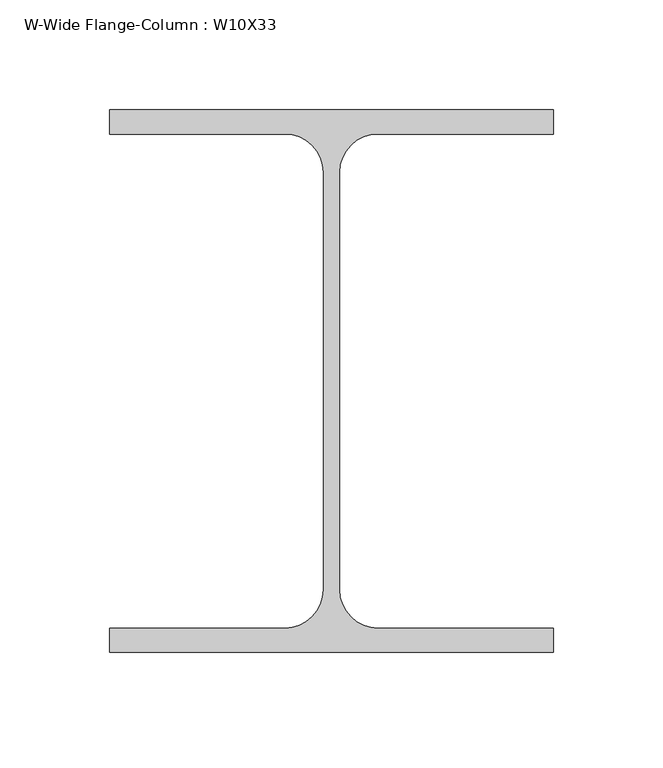
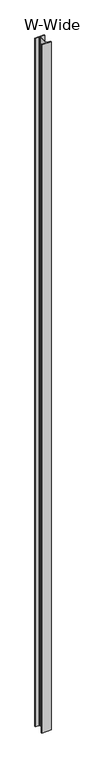
"""IFC4 building model written with IfcOpenShell, lengths in millimetres: column geometry, W-Wide Flange-Column : W10X33."""

import ifcopenshell
import ifcopenshell.guid

model = None  # the IFC model being written
_history = None  # IfcOwnerHistory: only IFC2X3 demands one
_inside = {}  # id of a spatial element -> (the spatial element, [elements in it])
_under = {}  # id of a project, library or spatial element -> (it, [spatial elements below it])
_declared = {}  # id of a project -> (the project, [libraries it declares])
_typed = {}  # id of a type object -> (the type object, [elements of that type])
_made_of = {}  # id of a material, layer set ... -> (it, [elements and type objects made of it])


def new_model(schema):
    """Start an empty IFC model of exactly this schema.

    Asked for "IFC4X3", IfcOpenShell would pick the latest addendum, in which some entities
    have other attributes; the version numbers below select the first issue.
    IFC2X3 requires an IfcOwnerHistory on every rooted entity: one is made here for all.
    """
    global model, _history
    if schema == "IFC4X3":
        model = ifcopenshell.file(schema_version=(4, 3, 0, 0))
    else:
        model = ifcopenshell.file(schema=schema)
    _inside.clear()
    _under.clear()
    _declared.clear()
    _typed.clear()
    _made_of.clear()
    _history = None
    if model.schema == "IFC2X3":
        org = make("IfcOrganization", Name="unknown")
        user = make(
            "IfcPersonAndOrganization",
            ThePerson=make("IfcPerson", FamilyName="unknown"),
            TheOrganization=org,
        )
        app = make(
            "IfcApplication",
            ApplicationDeveloper=org,
            Version="unknown",
            ApplicationFullName="unknown",
            ApplicationIdentifier="unknown",
        )
        _history = make(
            "IfcOwnerHistory",
            OwningUser=user,
            OwningApplication=app,
            ChangeAction="ADDED",
            CreationDate=0,
        )
    return model


def make(cls, **values):
    """One entity of the class cls with the attributes given. An attribute that is None is left unset."""
    return model.create_entity(
        cls, **{name: value for name, value in values.items() if value is not None}
    )


def rooted(cls, **values):
    """An entity with a GlobalId (a new one), such as an element, a storey or a relation."""
    return make(cls, GlobalId=ifcopenshell.guid.new(), OwnerHistory=_history, **values)


def si_unit(unit_type, name, prefix=None):
    """IfcSIUnit, for example si_unit("LENGTHUNIT", "METRE", prefix="MILLI")."""
    return make("IfcSIUnit", UnitType=unit_type, Prefix=prefix, Name=name)


def assignment(units):
    """IfcUnitAssignment: the units of a project."""
    return None if units is None else make("IfcUnitAssignment", Units=units)


def point(xyz):
    """IfcCartesianPoint."""
    return None if xyz is None else make("IfcCartesianPoint", Coordinates=xyz)


def direction(xyz):
    """IfcDirection."""
    return None if xyz is None else make("IfcDirection", DirectionRatios=xyz)


def frame(location, z_axis=None, x_axis=None):
    """IfcAxis2Placement3D, a coordinate frame: its origin and axes. An axis left out is left unset."""
    return make(
        "IfcAxis2Placement3D",
        Location=point(location),
        Axis=direction(z_axis),
        RefDirection=direction(x_axis),
    )


def frame_2d(location, x_axis=None):
    """IfcAxis2Placement2D, a coordinate frame in the plane: its origin and x axis."""
    return make(
        "IfcAxis2Placement2D", Location=point(location), RefDirection=direction(x_axis)
    )


def origin():
    """The frame at (0, 0, 0) with its axes left unset."""
    return frame((0.0, 0.0, 0.0))


def place(relative_to, where):
    """IfcLocalPlacement: puts the frame where relative to a parent placement (None: the world)."""
    return make(
        "IfcLocalPlacement", PlacementRelTo=relative_to, RelativePlacement=where
    )


def context(
    kind, dimensions, precision=None, world=None, true_north=None, identifier=None
):
    """IfcGeometricRepresentationContext, for example the 3D "Model" context."""
    return make(
        "IfcGeometricRepresentationContext",
        ContextIdentifier=identifier,
        ContextType=kind,
        CoordinateSpaceDimension=dimensions,
        Precision=precision,
        WorldCoordinateSystem=world,
        TrueNorth=true_north,
    )


def project(units=None, contexts=None):
    """IfcProject with its units and contexts."""
    return rooted(
        "IfcProject",
        Name="project",
        RepresentationContexts=contexts,
        UnitsInContext=assignment(units),
    )


def spatial(cls, under=None, at=None, **own):
    """A site, building, storey or space (cls), placed at a placement, below another one or the project."""
    s = rooted(cls, ObjectPlacement=at, **own)
    if under is not None:
        _under.setdefault(under.id(), (under, []))[1].append(s)
    return s


def polyline(points):
    """IfcPolyline through the points."""
    return make("IfcPolyline", Points=[point(p) for p in points])


def circle_curve(where, radius):
    """IfcCircle in the frame where."""
    return make("IfcCircle", Position=where, Radius=radius)


def trimmed(basis, trim1, trim2, sense, master):
    """IfcTrimmedCurve: the piece of a basis curve between two trims."""
    return make(
        "IfcTrimmedCurve",
        BasisCurve=basis,
        Trim1=trim1,
        Trim2=trim2,
        SenseAgreement=sense,
        MasterRepresentation=master,
    )


def segment(curve, same_sense, transition):
    """IfcCompositeCurveSegment."""
    return make(
        "IfcCompositeCurveSegment",
        Transition=transition,
        SameSense=same_sense,
        ParentCurve=curve,
    )


def composite_curve(segments, self_intersect=None):
    """IfcCompositeCurve: segments joined end to end."""
    return make("IfcCompositeCurve", Segments=segments, SelfIntersect=self_intersect)


def outline(outer, holes=None, kind="AREA"):
    """IfcArbitraryClosedProfileDef: a profile drawn as a closed curve; with holes, ...WithVoids."""
    if holes is None:
        return make("IfcArbitraryClosedProfileDef", ProfileType=kind, OuterCurve=outer)
    return make(
        "IfcArbitraryProfileDefWithVoids",
        ProfileType=kind,
        OuterCurve=outer,
        InnerCurves=holes,
    )


def extrude(swept, where, along, depth):
    """IfcExtrudedAreaSolid: the profile swept, set in the frame where, extruded along a direction by depth."""
    return make(
        "IfcExtrudedAreaSolid",
        SweptArea=swept,
        Position=where,
        ExtrudedDirection=direction(along),
        Depth=depth,
    )


def shape(context_of_items, identifier, shape_type, items):
    """IfcShapeRepresentation: the items that make up one representation, for example the "Body"."""
    return make(
        "IfcShapeRepresentation",
        ContextOfItems=context_of_items,
        RepresentationIdentifier=identifier,
        RepresentationType=shape_type,
        Items=items,
    )


def source(mapping_origin, context_of_items, identifier, shape_type, items):
    """IfcRepresentationMap: a shape defined once, which mapped items show again and again."""
    return make(
        "IfcRepresentationMap",
        MappingOrigin=mapping_origin,
        MappedRepresentation=shape(context_of_items, identifier, shape_type, items),
    )


def transform(
    local_origin,
    x_axis=None,
    y_axis=None,
    z_axis=None,
    scale=None,
    scale2=None,
    scale3=None,
    uniform=True,
):
    """IfcCartesianTransformationOperator3D, or its non-uniform kind. x_axis, y_axis, z_axis: its Axis1, 2, 3."""
    if uniform:
        return make(
            "IfcCartesianTransformationOperator3D",
            Axis1=direction(x_axis),
            Axis2=direction(y_axis),
            LocalOrigin=point(local_origin),
            Scale=scale,
            Axis3=direction(z_axis),
        )
    return make(
        "IfcCartesianTransformationOperator3DnonUniform",
        Axis1=direction(x_axis),
        Axis2=direction(y_axis),
        LocalOrigin=point(local_origin),
        Scale=scale,
        Axis3=direction(z_axis),
        Scale2=scale2,
        Scale3=scale3,
    )


def mapped(mapping_source, mapping_target):
    """IfcMappedItem: shows the shape of a source again, moved by a transform."""
    return make(
        "IfcMappedItem", MappingSource=mapping_source, MappingTarget=mapping_target
    )


def made_of(thing, what):
    """Note that an element or type object is made of a material, layer set ...; save() writes the relation."""
    if what is not None:
        _made_of.setdefault(what.id(), (what, []))[1].append(thing)
    return thing


def element(
    cls,
    number,
    at=None,
    inside=None,
    cuts=None,
    type_object=None,
    material=None,
    context=None,
    identifier="Body",
    shape_type=None,
    held_by="IfcProductDefinitionShape",
    body=None,
    shapes=None,
    **own,
):
    """One element of the class cls, such as IfcWall. Its Tag is "e" and its number.

    at: its placement. inside: the storey or other place that contains it. cuts: it is an
    opening in that element (IfcRelVoidsElement). A single representation is given by context,
    identifier, shape_type and body (its items); several are given by shapes. held_by: the class
    of the entity that holds the representations. save() writes the other relations.
    """
    e = rooted(cls, Tag="e%d" % number, ObjectPlacement=at, **own)
    if body is not None:
        shapes = [shape(context, identifier, shape_type, body)]
    if shapes is not None:
        e.Representation = make(held_by, Representations=shapes)
    if inside is not None:
        _inside.setdefault(inside.id(), (inside, []))[1].append(e)
    if cuts is not None:
        rooted(
            "IfcRelVoidsElement", RelatingBuildingElement=cuts, RelatedOpeningElement=e
        )
    if type_object is not None:
        _typed.setdefault(type_object.id(), (type_object, []))[1].append(e)
    return made_of(e, material)


def aggregate(whole, parts):
    """IfcRelAggregates: a whole, such as a stair, and the parts it consists of."""
    return rooted("IfcRelAggregates", RelatingObject=whole, RelatedObjects=parts)


def save(model, path):
    """Write the relations noted so far, then the file.

    IfcRelAggregates (storeys below a building ...), IfcRelContainedInSpatialStructure (elements
    in a storey), IfcRelDefinesByType, IfcRelAssociatesMaterial and IfcRelDeclares: one each for
    every whole, place, type object, material and project.
    """
    for whole, parts in _under.values():
        aggregate(whole, parts)
    for where, things in _inside.values():
        rooted(
            "IfcRelContainedInSpatialStructure",
            RelatedElements=things,
            RelatingStructure=where,
        )
    for kind, things in _typed.values():
        rooted("IfcRelDefinesByType", RelatedObjects=things, RelatingType=kind)
    for what, things in _made_of.values():
        rooted("IfcRelAssociatesMaterial", RelatedObjects=things, RelatingMaterial=what)
    for by, libraries in _declared.values():
        rooted("IfcRelDeclares", RelatingContext=by, RelatedDefinitions=libraries)
    model.write(path)


def w_wide_flange_column_w10x33_b445f528(model_context):
    return source(origin(), model_context, "Body", "SweptSolid", [
        extrude(outline(composite_curve([segment(polyline([(101.092, 123.571), (101.092, 112.522), (21.209, 112.522)]), True, "CONTINUOUS"), segment(trimmed(circle_curve(frame_2d((21.209, 94.996)), 17.526), [point((21.209, 112.522))], [point((3.683, 94.996))], True, "CARTESIAN"), True, "CONTINUOUS"), segment(polyline([(3.683, 94.996), (3.683, -94.996)]), True, "CONTINUOUS"), segment(trimmed(circle_curve(frame_2d((21.209, -94.996)), 17.526), [point((3.683, -94.996))], [point((21.209, -112.522))], True, "CARTESIAN"), True, "CONTINUOUS"), segment(polyline([(21.209, -112.522), (101.092, -112.522), (101.092, -123.571), (-101.092, -123.571), (-101.092, -112.522), (-21.209, -112.522)]), True, "CONTINUOUS"), segment(trimmed(circle_curve(frame_2d((-21.209, -94.996)), 17.526), [point((-21.209, -112.522))], [point((-3.683, -94.996))], True, "CARTESIAN"), True, "CONTINUOUS"), segment(polyline([(-3.683, -94.996), (-3.683, 94.996)]), True, "CONTINUOUS"), segment(trimmed(circle_curve(frame_2d((-21.209, 94.996)), 17.526), [point((-3.683, 94.996))], [point((-21.209, 112.522))], True, "CARTESIAN"), True, "CONTINUOUS"), segment(polyline([(-21.209, 112.522), (-101.092, 112.522), (-101.092, 123.571), (101.092, 123.571)]), True, "CONTINUOUS")], self_intersect=False)), frame((0.0, 0.0, 8756.65), z_axis=(0.0, 0.0, 1.0), x_axis=(1.0, 0.0, 0.0)), (0.0, 0.0, 1.0), 15584.1898438),
    ])


if __name__ == "__main__":
    model = new_model("IFC4")
    model_context = context("Model", 3, world=origin())
    ifc_project = project(units=[si_unit("LENGTHUNIT", "METRE", prefix="MILLI")], contexts=[model_context])
    site = spatial("IfcSite", under=ifc_project)
    building = spatial("IfcBuilding", under=site)
    placement = place(None, origin())
    w_wide_flange_column_w10x33_shape = w_wide_flange_column_w10x33_b445f528(model_context)
    element("IfcColumn", 1, ObjectType="W-Wide Flange-Column : W10X33", at=placement, inside=building, context=model_context, shape_type="MappedRepresentation", body=[
        mapped(w_wide_flange_column_w10x33_shape, transform((0.0, 0.0, 0.0), x_axis=(1.0, 0.0, 0.0), y_axis=(0.0, 1.0, 0.0), z_axis=(0.0, 0.0, 1.0))),
    ])
    save(model, "model.ifc")

# Revit data of these elements
# Type "W-Wide Flange-Column : W10X33"
#   Assembly Code = "B10"
#   W = 33
#   bf = 0' - 7.96"
#   d = 0' - 9.73"
#   k = 0' - 1 1/8"
#   kr = 0' - 0.69"
#   tf = 0' - 0.435"
#   tw = 0' - 0.29"
#   A = 0.0674306 SF
#   Structural Material [instance default] = Steel ASTM A992
# Element 1 (IfcColumn, "W-Wide Flange-Column : W10X33")
#   Materials on its faces: "Steel ASTM A992"
# Materials
#   "Steel ASTM A992": class "Metal", colour RGB 199 199 199, transparency 0, Description = "Structural steel 50ksi", Cost = 0
